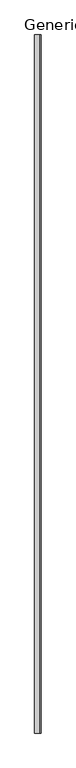
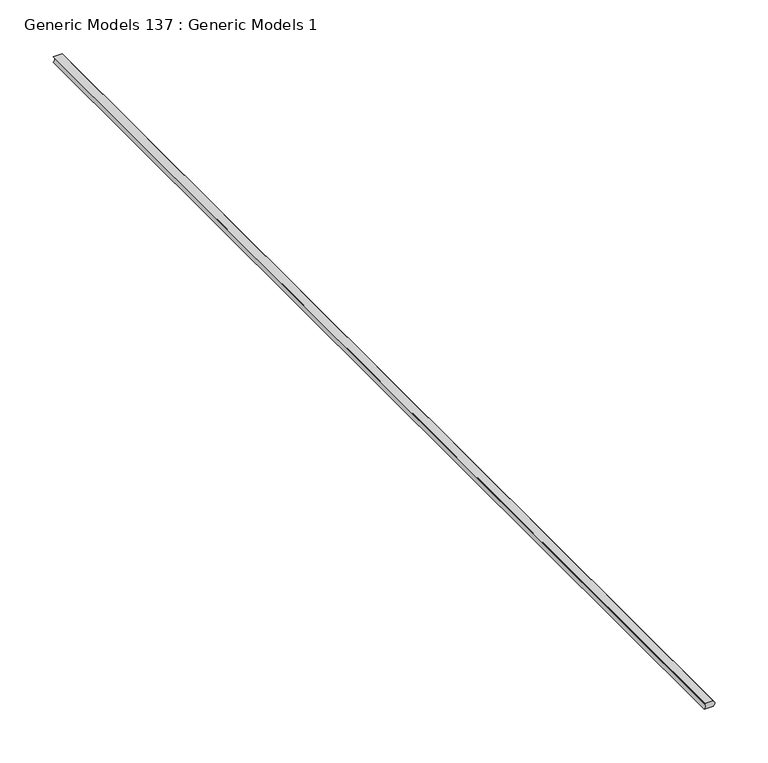
"""IFC4 building model written with IfcOpenShell, lengths in millimetres: proxy geometry, Generic Models 137 : Generic Models 1."""

from ifc_helpers import new_model, si_unit, point, frame, frame_2d, origin, place, context, project, spatial, polyline, circle_curve, trimmed, segment, composite_curve, outline, extrude, source, transform, mapped, element, save


def generic_models_137_generic_models_1_9cb7df0c(model_context):
    return source(origin(), model_context, "Body", "SweptSolid", [
        extrude(outline(composite_curve([segment(polyline([(-225.976067, 48050.3548058), (-225.976067, 48059.8798058)]), True, "CONTINUOUS"), segment(trimmed(circle_curve(frame_2d((-222.801067, 48056.9650653)), 4.3100275), [point((-225.976067, 48059.8798058))], [point((-219.626067, 48059.8798058))], False, "CARTESIAN"), True, "CONTINUOUS"), segment(polyline([(-219.626067, 48059.8798058), (-219.626067, 48050.3548058)]), True, "CONTINUOUS"), segment(trimmed(circle_curve(frame_2d((-222.801067, 48047.4400653)), 4.3100275), [point((-219.626067, 48050.3548058))], [point((-225.976067, 48050.3548058))], True, "CARTESIAN"), True, "CONTINUOUS")], self_intersect=False)), frame((0.0, 0.0, 0.0), z_axis=(0.0, 1.0, 0.0), x_axis=(0.0, 0.0, 1.0)), (0.0, 0.0, 1.0), 1219.2),
    ])


if __name__ == "__main__":
    model = new_model("IFC4")
    model_context = context("Model", 3, world=origin())
    ifc_project = project(units=[si_unit("LENGTHUNIT", "METRE", prefix="MILLI")], contexts=[model_context])
    site = spatial("IfcSite", under=ifc_project)
    building = spatial("IfcBuilding", under=site)
    placement = place(None, origin())
    generic_models_137_generic_models_1_shape = generic_models_137_generic_models_1_9cb7df0c(model_context)
    element("IfcBuildingElementProxy", 1, Name="Generic Models 137 : Generic Models 1", ObjectType="Generic Models 137 : Generic Models 1", at=placement, inside=building, context=model_context, shape_type="MappedRepresentation", body=[
        mapped(generic_models_137_generic_models_1_shape, transform((0.0, 0.0, 0.0), x_axis=(1.0, 0.0, 0.0), y_axis=(0.0, 1.0, 0.0), z_axis=(0.0, 0.0, 1.0))),
    ])
    save(model, "model.ifc")

# Revit data of these elements
# Element 1 (IfcBuildingElementProxy, "Generic Models 137 : Generic Models 1")
#   Materials on its faces: "SEALANT (W/ BACKER ROD IF NECESSARY)"
# Materials
#   "SEALANT (W/ BACKER ROD IF NECESSARY)": class "Unassigned", colour RGB 120 120 120, transparency 0, Cost = 0
